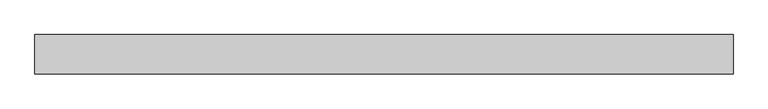
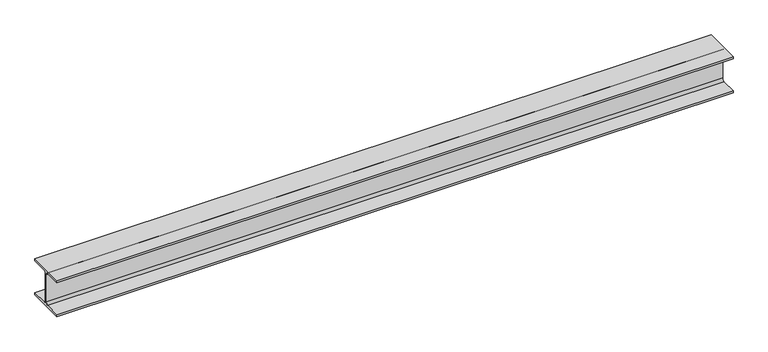
"""IFC4 building model written with IfcOpenShell, lengths in millimetres: beam geometry, 0912_Steel Framing_H-KSD3502 : H_SB_ASB_H-200x200x8x12."""

from ifc_helpers import new_model, si_unit, point, frame, frame_2d, origin, place, context, project, spatial, polyline, circle_curve, trimmed, segment, composite_curve, outline, extrude, source, transform, mapped, element, save


def beam_d67612f9(model_context):
    return source(origin(), model_context, "Body", "SweptSolid", [
        extrude(outline(composite_curve([segment(polyline([(100.0, -88.0), (100.0, -100.0), (-100.0, -100.0), (-100.0, -88.0), (-17.0, -88.0)]), True, "CONTINUOUS"), segment(trimmed(circle_curve(frame_2d((-17.0, -75.0)), 13.0), [point((-17.0, -88.0))], [point((-4.0, -75.0))], True, "CARTESIAN"), True, "CONTINUOUS"), segment(polyline([(-4.0, -75.0), (-4.0, 75.0)]), True, "CONTINUOUS"), segment(trimmed(circle_curve(frame_2d((-17.0, 75.0)), 13.0), [point((-4.0, 75.0))], [point((-17.0, 88.0))], True, "CARTESIAN"), True, "CONTINUOUS"), segment(polyline([(-17.0, 88.0), (-100.0, 88.0), (-100.0, 100.0), (100.0, 100.0), (100.0, 88.0), (17.0, 88.0)]), True, "CONTINUOUS"), segment(trimmed(circle_curve(frame_2d((17.0, 75.0)), 13.0), [point((17.0, 88.0))], [point((4.0, 75.0))], True, "CARTESIAN"), True, "CONTINUOUS"), segment(polyline([(4.0, 75.0), (4.0, -75.0)]), True, "CONTINUOUS"), segment(trimmed(circle_curve(frame_2d((17.0, -75.0)), 13.0), [point((4.0, -75.0))], [point((17.0, -88.0))], True, "CARTESIAN"), True, "CONTINUOUS"), segment(polyline([(17.0, -88.0), (100.0, -88.0)]), True, "CONTINUOUS")], self_intersect=False)), frame((-1868.2054994, 0.0, 0.0), z_axis=(1.0, 0.0, 0.0), x_axis=(0.0, 1.0, 0.0)), (0.0, 0.0, 1.0), 3550.9309259),
    ])


if __name__ == "__main__":
    model = new_model("IFC4")
    model_context = context("Model", 3, world=origin())
    ifc_project = project(units=[si_unit("LENGTHUNIT", "METRE", prefix="MILLI")], contexts=[model_context])
    site = spatial("IfcSite", under=ifc_project)
    building = spatial("IfcBuilding", under=site)
    placement = place(None, origin())
    beam_shape = beam_d67612f9(model_context)
    element("IfcBeam", 1, ObjectType="0912_Steel Framing_H-KSD3502 : H_SB_ASB_H-200x200x8x12", at=placement, inside=building, context=model_context, shape_type="MappedRepresentation", body=[
        mapped(beam_shape, transform((0.0, 0.0, 0.0), x_axis=(1.0, 0.0, 0.0), y_axis=(0.0, 1.0, 0.0), z_axis=(0.0, 0.0, 1.0))),
    ])
    save(model, "model.ifc")

# Revit data of these elements
# Type "0912_Steel Framing_H-KSD3502 : H_SB_ASB_H-200x200x8x12"
#   H_WM Code_1 = "S01AA002-00001 | Main Steel Structure Fabrication Work | Shelter/Building | Medium Steel - Standard (90KG/M>Weight≥30KG/M) | Material: (   )"
#   H_WM Code_2 = "S03AA028-00001 | Main Steel Structure Erection Work | Shelter/Building | Medium Steel (90KG/M>Weight≥30KG/M) | Material: (   )"
#   H_WM Code_3 = "S01AA010-00001 | Main Steel Structure Fabrication Work | Shelter/Building | Steel Painting/Coating | for Non-Fireproofed Steel Surface, Surface Preparation, Primer, Second & Final Coat | Material: (   )"
#   H_Q'ty Cal Type Tag = "SB-Q2"
#   Width = 20.0 cm
#   Web Thickness = 0.8 cm
#   Web Fillet = 1.3 cm
#   Warping Constant = 141000.0 cm⁶
#   W = 0
#   Torsional Moment of Inertia = 26.2485 cm⁴
#   Section Area = 63.53 cm²
#   Plastic Modulus weak axis = 244.0 cm³
#   Plastic Modulus strong axis = 525.0 cm³
#   Perimeter = 1.16 m²/m
#   Nominal Weight = 49.90 kgf/m
#   Moment of Inertia weak axis = 1600.00 cm⁴
#   Moment of Inertia strong axis = 4720.00 cm⁴
#   Height = 20.0 cm
#   Flange Thickness = 1.2 cm
#   Elastic Modulus weak axis = 160.0 cm³
#   Elastic Modulus strong axis = 472.0 cm³
#   Centroid Vertical = 10.0 cm
#   Centroid Horizontal = 10.0 cm
#   Ix = 47200000
#   Length [instance default] = 1.5240 m
#   Zx = 525000
#   b = 0.2000 m
#   h = 0.2000 m
#   r = 0.0130 m
#   s = 0.0080 m
#   t = 0.0120 m
#   A = 0.006353 m²
#   Structural Material [instance default] = Steel, 45-345
#   Assembly Code = ""
# Element 1 (IfcBeam, "0912_Steel Framing_H-KSD3502 : H_SB_ASB_H-200x200x8x12")
#   Structural Material = none
# Materials
#   "Steel, 45-345": class "Metal", colour RGB 189 187 185, transparency 0, Description = "Steel 345 MPa", Cost = 0
